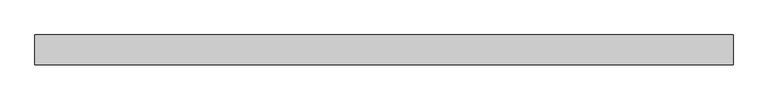
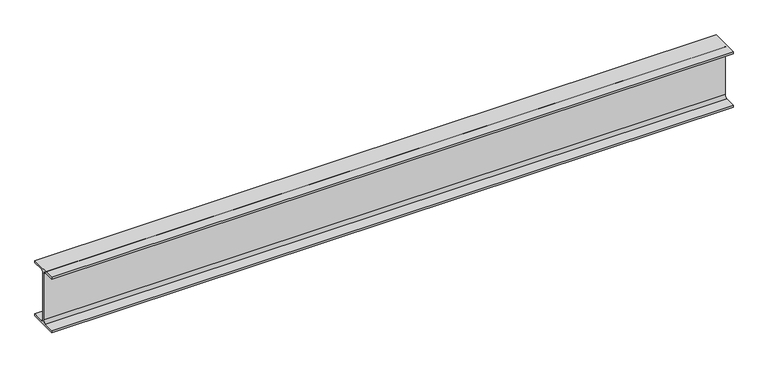
"""IFC4 building model written with IfcOpenShell, lengths in millimetres: beam geometry, 0912_Steel Framing_H-KSD3502 : H_SB_ASB_H-250x125x6x9."""

from ifc_helpers import new_model, si_unit, point, frame, frame_2d, origin, place, context, project, spatial, polyline, circle_curve, trimmed, segment, composite_curve, outline, extrude, source, transform, mapped, element, save


def beam_ab81005f(model_context):
    return source(origin(), model_context, "Body", "SweptSolid", [
        extrude(outline(composite_curve([segment(polyline([(62.5, -116.0), (62.5, -125.0), (-62.5, -125.0), (-62.5, -116.0), (-15.0, -116.0)]), True, "CONTINUOUS"), segment(trimmed(circle_curve(frame_2d((-15.0, -104.0)), 12.0), [point((-15.0, -116.0))], [point((-3.0, -104.0))], True, "CARTESIAN"), True, "CONTINUOUS"), segment(polyline([(-3.0, -104.0), (-3.0, 104.0)]), True, "CONTINUOUS"), segment(trimmed(circle_curve(frame_2d((-15.0, 104.0)), 12.0), [point((-3.0, 104.0))], [point((-15.0, 116.0))], True, "CARTESIAN"), True, "CONTINUOUS"), segment(polyline([(-15.0, 116.0), (-62.5, 116.0), (-62.5, 125.0), (62.5, 125.0), (62.5, 116.0), (15.0, 116.0)]), True, "CONTINUOUS"), segment(trimmed(circle_curve(frame_2d((15.0, 104.0)), 12.0), [point((15.0, 116.0))], [point((3.0, 104.0))], True, "CARTESIAN"), True, "CONTINUOUS"), segment(polyline([(3.0, 104.0), (3.0, -104.0)]), True, "CONTINUOUS"), segment(trimmed(circle_curve(frame_2d((15.0, -104.0)), 12.0), [point((3.0, -104.0))], [point((15.0, -116.0))], True, "CARTESIAN"), True, "CONTINUOUS"), segment(polyline([(15.0, -116.0), (62.5, -116.0)]), True, "CONTINUOUS")], self_intersect=False)), frame((-1529.8000466, 0.0, 0.0), z_axis=(1.0, 0.0, 0.0), x_axis=(0.0, 1.0, 0.0)), (0.0, 0.0, 1.0), 2912.0982036),
    ])


if __name__ == "__main__":
    model = new_model("IFC4")
    model_context = context("Model", 3, world=origin())
    ifc_project = project(units=[si_unit("LENGTHUNIT", "METRE", prefix="MILLI")], contexts=[model_context])
    site = spatial("IfcSite", under=ifc_project)
    building = spatial("IfcBuilding", under=site)
    placement = place(None, origin())
    beam_shape = beam_ab81005f(model_context)
    element("IfcBeam", 1, ObjectType="0912_Steel Framing_H-KSD3502 : H_SB_ASB_H-250x125x6x9", at=placement, inside=building, context=model_context, shape_type="MappedRepresentation", body=[
        mapped(beam_shape, transform((0.0, 0.0, 0.0), x_axis=(1.0, 0.0, 0.0), y_axis=(0.0, 1.0, 0.0), z_axis=(0.0, 0.0, 1.0))),
    ])
    save(model, "model.ifc")

# Revit data of these elements
# Type "0912_Steel Framing_H-KSD3502 : H_SB_ASB_H-250x125x6x9"
#   H_WM Code_1 = "S01AA003-00001 | Main Steel Structure Fabrication Work | Shelter/Building | Light Steel - Standard (30KG/M>Weight) | Material: (   )"
#   H_WM Code_2 = "S03AA029-00001 | Main Steel Structure Erection Work | Shelter/Building | Light Steel (30KG/M>Weight) | Material: (   )"
#   H_WM Code_3 = "S01AA010-00001 | Main Steel Structure Fabrication Work | Shelter/Building | Steel Painting/Coating | for Non-Fireproofed Steel Surface, Surface Preparation, Primer, Second & Final Coat | Material: (   )"
#   H_Q'ty Cal Type Tag = "SB-Q2"
#   Width = 12.5 cm
#   Web Thickness = 0.6 cm
#   Web Fillet = 1.2 cm
#   Warping Constant = 42539.8 cm⁶
#   W = 0
#   Torsional Moment of Inertia = 7.8102 cm⁴
#   Section Area = 37.66 cm²
#   Plastic Modulus weak axis = 73.1 cm³
#   Plastic Modulus strong axis = 366.0 cm³
#   Perimeter = 0.97 m²/m
#   Nominal Weight = 29.60 kgf/m
#   Moment of Inertia weak axis = 294.00 cm⁴
#   Moment of Inertia strong axis = 4050.00 cm⁴
#   Height = 25.0 cm
#   Flange Thickness = 0.9 cm
#   Elastic Modulus weak axis = 47.0 cm³
#   Elastic Modulus strong axis = 324.0 cm³
#   Centroid Vertical = 12.5 cm
#   Centroid Horizontal = 6.25 cm
#   Ix = 40500000
#   Length [instance default] = 1.5240 m
#   Zx = 366000
#   b = 0.1250 m
#   h = 0.2500 m
#   r = 0.0120 m
#   s = 0.0060 m
#   t = 0.0090 m
#   A = 0.003766 m²
#   Structural Material [instance default] = Steel, 45-345
#   Assembly Code = ""
# Element 1 (IfcBeam, "0912_Steel Framing_H-KSD3502 : H_SB_ASB_H-250x125x6x9")
#   Structural Material = none
# Materials
#   "Steel, 45-345": class "Metal", colour RGB 189 187 185, transparency 0, Description = "Steel 345 MPa", Cost = 0
